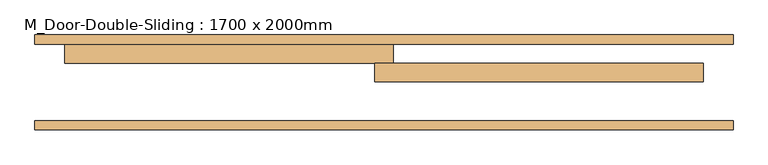
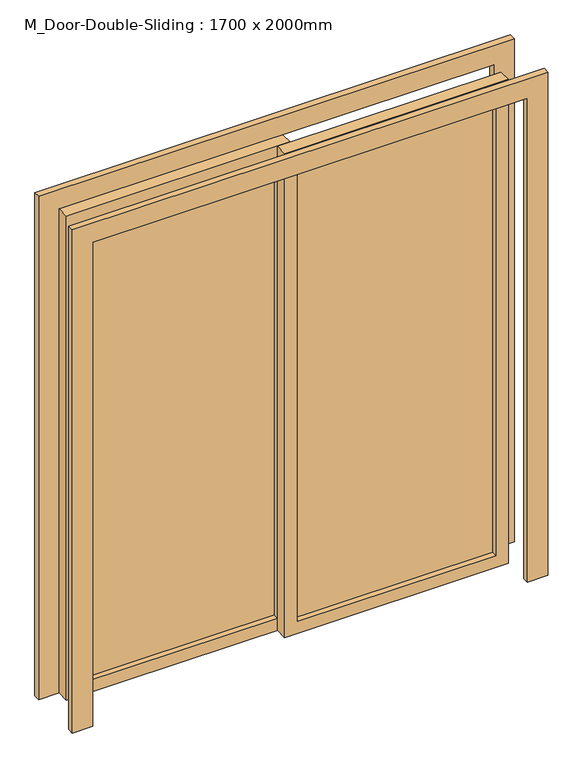
"""IFC4 building model written with IfcOpenShell, lengths in millimetres: door geometry, M_Door-Double-Sliding : 1700 x 2000mm."""

import ifcopenshell
import ifcopenshell.guid

model = None  # the IFC model being written
_history = None  # IfcOwnerHistory: only IFC2X3 demands one
_inside = {}  # id of a spatial element -> (the spatial element, [elements in it])
_under = {}  # id of a project, library or spatial element -> (it, [spatial elements below it])
_declared = {}  # id of a project -> (the project, [libraries it declares])
_typed = {}  # id of a type object -> (the type object, [elements of that type])
_made_of = {}  # id of a material, layer set ... -> (it, [elements and type objects made of it])


def new_model(schema):
    """Start an empty IFC model of exactly this schema.

    Asked for "IFC4X3", IfcOpenShell would pick the latest addendum, in which some entities
    have other attributes; the version numbers below select the first issue.
    IFC2X3 requires an IfcOwnerHistory on every rooted entity: one is made here for all.
    """
    global model, _history
    if schema == "IFC4X3":
        model = ifcopenshell.file(schema_version=(4, 3, 0, 0))
    else:
        model = ifcopenshell.file(schema=schema)
    _inside.clear()
    _under.clear()
    _declared.clear()
    _typed.clear()
    _made_of.clear()
    _history = None
    if model.schema == "IFC2X3":
        org = make("IfcOrganization", Name="unknown")
        user = make(
            "IfcPersonAndOrganization",
            ThePerson=make("IfcPerson", FamilyName="unknown"),
            TheOrganization=org,
        )
        app = make(
            "IfcApplication",
            ApplicationDeveloper=org,
            Version="unknown",
            ApplicationFullName="unknown",
            ApplicationIdentifier="unknown",
        )
        _history = make(
            "IfcOwnerHistory",
            OwningUser=user,
            OwningApplication=app,
            ChangeAction="ADDED",
            CreationDate=0,
        )
    return model


def make(cls, **values):
    """One entity of the class cls with the attributes given. An attribute that is None is left unset."""
    return model.create_entity(
        cls, **{name: value for name, value in values.items() if value is not None}
    )


def rooted(cls, **values):
    """An entity with a GlobalId (a new one), such as an element, a storey or a relation."""
    return make(cls, GlobalId=ifcopenshell.guid.new(), OwnerHistory=_history, **values)


def si_unit(unit_type, name, prefix=None):
    """IfcSIUnit, for example si_unit("LENGTHUNIT", "METRE", prefix="MILLI")."""
    return make("IfcSIUnit", UnitType=unit_type, Prefix=prefix, Name=name)


def assignment(units):
    """IfcUnitAssignment: the units of a project."""
    return None if units is None else make("IfcUnitAssignment", Units=units)


def point(xyz):
    """IfcCartesianPoint."""
    return None if xyz is None else make("IfcCartesianPoint", Coordinates=xyz)


def direction(xyz):
    """IfcDirection."""
    return None if xyz is None else make("IfcDirection", DirectionRatios=xyz)


def frame(location, z_axis=None, x_axis=None):
    """IfcAxis2Placement3D, a coordinate frame: its origin and axes. An axis left out is left unset."""
    return make(
        "IfcAxis2Placement3D",
        Location=point(location),
        Axis=direction(z_axis),
        RefDirection=direction(x_axis),
    )


def origin():
    """The frame at (0, 0, 0) with its axes left unset."""
    return frame((0.0, 0.0, 0.0))


def place(relative_to, where):
    """IfcLocalPlacement: puts the frame where relative to a parent placement (None: the world)."""
    return make(
        "IfcLocalPlacement", PlacementRelTo=relative_to, RelativePlacement=where
    )


def context(
    kind, dimensions, precision=None, world=None, true_north=None, identifier=None
):
    """IfcGeometricRepresentationContext, for example the 3D "Model" context."""
    return make(
        "IfcGeometricRepresentationContext",
        ContextIdentifier=identifier,
        ContextType=kind,
        CoordinateSpaceDimension=dimensions,
        Precision=precision,
        WorldCoordinateSystem=world,
        TrueNorth=true_north,
    )


def project(units=None, contexts=None):
    """IfcProject with its units and contexts."""
    return rooted(
        "IfcProject",
        Name="project",
        RepresentationContexts=contexts,
        UnitsInContext=assignment(units),
    )


def spatial(cls, under=None, at=None, **own):
    """A site, building, storey or space (cls), placed at a placement, below another one or the project."""
    s = rooted(cls, ObjectPlacement=at, **own)
    if under is not None:
        _under.setdefault(under.id(), (under, []))[1].append(s)
    return s


def polyline(points):
    """IfcPolyline through the points."""
    return make("IfcPolyline", Points=[point(p) for p in points])


def outline(outer, holes=None, kind="AREA"):
    """IfcArbitraryClosedProfileDef: a profile drawn as a closed curve; with holes, ...WithVoids."""
    if holes is None:
        return make("IfcArbitraryClosedProfileDef", ProfileType=kind, OuterCurve=outer)
    return make(
        "IfcArbitraryProfileDefWithVoids",
        ProfileType=kind,
        OuterCurve=outer,
        InnerCurves=holes,
    )


def extrude(swept, where, along, depth):
    """IfcExtrudedAreaSolid: the profile swept, set in the frame where, extruded along a direction by depth."""
    return make(
        "IfcExtrudedAreaSolid",
        SweptArea=swept,
        Position=where,
        ExtrudedDirection=direction(along),
        Depth=depth,
    )


def shape(context_of_items, identifier, shape_type, items):
    """IfcShapeRepresentation: the items that make up one representation, for example the "Body"."""
    return make(
        "IfcShapeRepresentation",
        ContextOfItems=context_of_items,
        RepresentationIdentifier=identifier,
        RepresentationType=shape_type,
        Items=items,
    )


def source(mapping_origin, context_of_items, identifier, shape_type, items):
    """IfcRepresentationMap: a shape defined once, which mapped items show again and again."""
    return make(
        "IfcRepresentationMap",
        MappingOrigin=mapping_origin,
        MappedRepresentation=shape(context_of_items, identifier, shape_type, items),
    )


def transform(
    local_origin,
    x_axis=None,
    y_axis=None,
    z_axis=None,
    scale=None,
    scale2=None,
    scale3=None,
    uniform=True,
):
    """IfcCartesianTransformationOperator3D, or its non-uniform kind. x_axis, y_axis, z_axis: its Axis1, 2, 3."""
    if uniform:
        return make(
            "IfcCartesianTransformationOperator3D",
            Axis1=direction(x_axis),
            Axis2=direction(y_axis),
            LocalOrigin=point(local_origin),
            Scale=scale,
            Axis3=direction(z_axis),
        )
    return make(
        "IfcCartesianTransformationOperator3DnonUniform",
        Axis1=direction(x_axis),
        Axis2=direction(y_axis),
        LocalOrigin=point(local_origin),
        Scale=scale,
        Axis3=direction(z_axis),
        Scale2=scale2,
        Scale3=scale3,
    )


def mapped(mapping_source, mapping_target):
    """IfcMappedItem: shows the shape of a source again, moved by a transform."""
    return make(
        "IfcMappedItem", MappingSource=mapping_source, MappingTarget=mapping_target
    )


def made_of(thing, what):
    """Note that an element or type object is made of a material, layer set ...; save() writes the relation."""
    if what is not None:
        _made_of.setdefault(what.id(), (what, []))[1].append(thing)
    return thing


def element(
    cls,
    number,
    at=None,
    inside=None,
    cuts=None,
    type_object=None,
    material=None,
    context=None,
    identifier="Body",
    shape_type=None,
    held_by="IfcProductDefinitionShape",
    body=None,
    shapes=None,
    **own,
):
    """One element of the class cls, such as IfcWall. Its Tag is "e" and its number.

    at: its placement. inside: the storey or other place that contains it. cuts: it is an
    opening in that element (IfcRelVoidsElement). A single representation is given by context,
    identifier, shape_type and body (its items); several are given by shapes. held_by: the class
    of the entity that holds the representations. save() writes the other relations.
    """
    e = rooted(cls, Tag="e%d" % number, ObjectPlacement=at, **own)
    if body is not None:
        shapes = [shape(context, identifier, shape_type, body)]
    if shapes is not None:
        e.Representation = make(held_by, Representations=shapes)
    if inside is not None:
        _inside.setdefault(inside.id(), (inside, []))[1].append(e)
    if cuts is not None:
        rooted(
            "IfcRelVoidsElement", RelatingBuildingElement=cuts, RelatedOpeningElement=e
        )
    if type_object is not None:
        _typed.setdefault(type_object.id(), (type_object, []))[1].append(e)
    return made_of(e, material)


def aggregate(whole, parts):
    """IfcRelAggregates: a whole, such as a stair, and the parts it consists of."""
    return rooted("IfcRelAggregates", RelatingObject=whole, RelatedObjects=parts)


def save(model, path):
    """Write the relations noted so far, then the file.

    IfcRelAggregates (storeys below a building ...), IfcRelContainedInSpatialStructure (elements
    in a storey), IfcRelDefinesByType, IfcRelAssociatesMaterial and IfcRelDeclares: one each for
    every whole, place, type object, material and project.
    """
    for whole, parts in _under.values():
        aggregate(whole, parts)
    for where, things in _inside.values():
        rooted(
            "IfcRelContainedInSpatialStructure",
            RelatedElements=things,
            RelatingStructure=where,
        )
    for kind, things in _typed.values():
        rooted("IfcRelDefinesByType", RelatedObjects=things, RelatingType=kind)
    for what, things in _made_of.values():
        rooted("IfcRelAssociatesMaterial", RelatedObjects=things, RelatingMaterial=what)
    for by, libraries in _declared.values():
        rooted("IfcRelDeclares", RelatingContext=by, RelatedDefinitions=libraries)
    model.write(path)


def m_door_double_sliding_1700_x_2000mm_96dae475(model_context):
    return source(origin(), model_context, "Body", "SweptSolid", [
        extrude(outline(polyline([(0.0, -930.0), (0.0, -850.0), (2000.0, -850.0), (2000.0, 850.0), (0.0, 850.0), (0.0, 930.0), (2080.0, 930.0), (2080.0, -930.0), (0.0, -930.0)])), frame((0.0, 0.4, 0.0), z_axis=(0.0, 1.0, 0.0), x_axis=(0.0, 0.0, 1.0)), (0.0, 0.0, 1.0), 25.0),
        extrude(outline(polyline([(0.0, 930.0), (2080.0, 930.0), (2080.0, -930.0), (0.0, -930.0), (0.0, -850.0), (2000.0, -850.0), (2000.0, 850.0), (0.0, 850.0), (0.0, 930.0)])), frame((0.0, 228.6, 0.0), z_axis=(0.0, 1.0, 0.0), x_axis=(0.0, 0.0, 1.0)), (0.0, 0.0, 1.0), 25.0),
        extrude(outline(polyline([(2000.0, -25.0), (0.0, -25.0), (0.0, 850.0), (2000.0, 850.0), (2000.0, -25.0)]), holes=[polyline([(1950.0, 25.0), (1950.0, 800.0), (50.0, 800.0), (50.0, 25.0), (1950.0, 25.0)])]), frame((0.0, 128.6, 0.0), z_axis=(0.0, 1.0, 0.0), x_axis=(0.0, 0.0, 1.0)), (0.0, 0.0, 1.0), 50.0),
        extrude(outline(polyline([(2000.0, 25.0), (2000.0, -850.0), (0.0, -850.0), (0.0, 25.0), (2000.0, 25.0)]), holes=[polyline([(1950.0, -25.0), (50.0, -25.0), (50.0, -800.0), (1950.0, -800.0), (1950.0, -25.0)])]), frame((0.0, 178.6, 0.0), z_axis=(0.0, 1.0, 0.0), x_axis=(0.0, 0.0, 1.0)), (0.0, 0.0, 1.0), 50.0),
        extrude(outline(polyline([(25.0, 156.775), (800.0, 156.775), (800.0, 150.425), (25.0, 150.425), (25.0, 156.775)])), frame((0.0, 0.0, 50.0), z_axis=(0.0, 0.0, 1.0), x_axis=(1.0, 0.0, 0.0)), (0.0, 0.0, 1.0), 1900.0),
        extrude(outline(polyline([(-25.0, 200.025), (-800.0, 200.025), (-800.0, 206.375), (-25.0, 206.375), (-25.0, 200.025)])), frame((0.0, 0.0, 50.0), z_axis=(0.0, 0.0, 1.0), x_axis=(1.0, 0.0, 0.0)), (0.0, 0.0, 1.0), 1900.0),
    ])


if __name__ == "__main__":
    model = new_model("IFC4")
    model_context = context("Model", 3, world=origin())
    ifc_project = project(units=[si_unit("LENGTHUNIT", "METRE", prefix="MILLI")], contexts=[model_context])
    site = spatial("IfcSite", under=ifc_project)
    building = spatial("IfcBuilding", under=site)
    placement = place(None, origin())
    m_door_double_sliding_1700_x_2000mm_shape = m_door_double_sliding_1700_x_2000mm_96dae475(model_context)
    element("IfcDoor", 1, ObjectType="M_Door-Double-Sliding : 1700 x 2000mm", at=placement, inside=building, context=model_context, shape_type="MappedRepresentation", body=[
        mapped(m_door_double_sliding_1700_x_2000mm_shape, transform((0.0, 0.0, 0.0), x_axis=(1.0, 0.0, 0.0), y_axis=(0.0, 1.0, 0.0), z_axis=(0.0, 0.0, 1.0))),
    ])
    save(model, "model.ifc")

# Revit data of these elements
# Type "M_Door-Double-Sliding : 1700 x 2000mm"
#   Type Mark = "11"
#   Construction Type Id = "opn-d45"
#   Assembly Code = "C1020"
#   Analytic Construction = "Wood frame, double glass door "
#   Thickness = 0' - 1.9685"
#   Thermal Resistance (R) = 0.31964 (m²·K)/W
#   Heat Transfer Coefficient (U) = 3.12872 W/(m²·K)
#   Height = 6' - 6.74016"
#   Rail Width = 0' - 1.9685"
#   Stiles = 0' - 1.9685"
#   Trim Projection Ext = 0' - 0.98425"
#   Trim Projection Int = 0' - 0.98425"
#   Trim Width = 0' - 3.14961"
#   Width = 5' - 6.92913"
#   Glazing = Glass
#   Panel Material = Wood - Birch - Solid Stained Light Low Gloss
#   Trim Material = Paint - Sienna
#   Visual Light Transmittance = 0
#   Solar Heat Gain Coefficient = 0
#   Function = (empty or 0)
#   Wall Closure = (empty or 0)
# Element 1 (IfcDoor, "M_Door-Double-Sliding : 1700 x 2000mm")
#   Materials on its faces: "Paint - Sienna", "Wood - Birch - Solid Stained Light Low Gloss", "Glass"
# Materials
#   "Glass": class "Glass", colour RGB 0 128 192, transparency 0.75, Description = "Soda Lime Glass", Cost = 0
#   "Wood - Birch - Solid Stained Light Low Gloss": class "Wood", colour RGB 210 159 95, transparency 0, Cost = 0
#   "Paint - Sienna": class "Miscellaneous", colour RGB 118 70 51, transparency 0, Cost = 0
